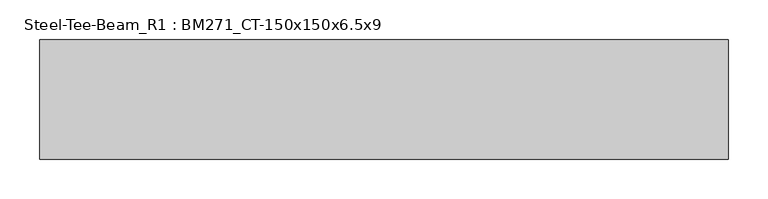
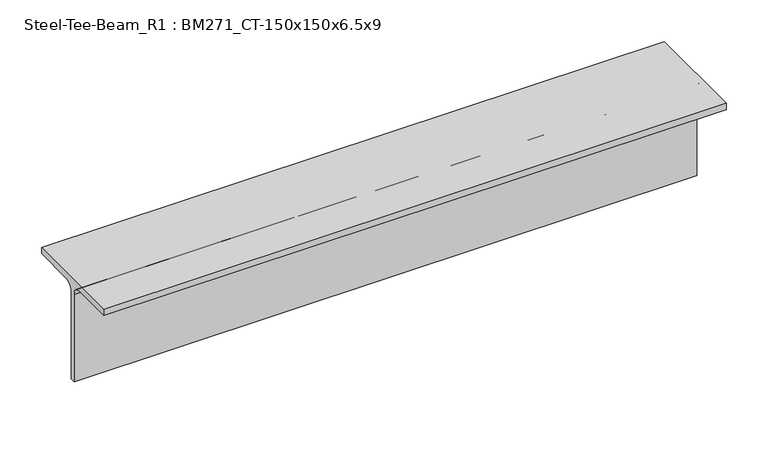
"""IFC4 building model written with IfcOpenShell, lengths in millimetres: member geometry, Steel-Tee-Beam_R1 : BM271_CT-150x150x6.5x9."""

from ifc_helpers import new_model, si_unit, point, frame, frame_2d, origin, place, context, project, spatial, polyline, circle_curve, trimmed, segment, composite_curve, outline, extrude, source, transform, mapped, element, save


def steel_tee_beam_r1_bm271_ct_150x150x6_5x9_bb86e743(model_context):
    return source(origin(), model_context, "Body", "SweptSolid", [
        extrude(outline(composite_curve([segment(polyline([(-75.0, 75.0), (75.0, 75.0), (75.0, 66.0), (16.25, 66.0)]), True, "CONTINUOUS"), segment(trimmed(circle_curve(frame_2d((16.25, 53.0)), 13.0), [point((16.25, 66.0))], [point((3.25, 53.0))], True, "CARTESIAN"), True, "CONTINUOUS"), segment(polyline([(3.25, 53.0), (3.25, -75.0), (-3.25, -75.0), (-3.25, 53.0)]), True, "CONTINUOUS"), segment(trimmed(circle_curve(frame_2d((-16.25, 53.0)), 13.0), [point((-3.25, 53.0))], [point((-16.25, 66.0))], True, "CARTESIAN"), True, "CONTINUOUS"), segment(polyline([(-16.25, 66.0), (-75.0, 66.0), (-75.0, 75.0)]), True, "CONTINUOUS")], self_intersect=False)), frame((-500.0, 0.0, 0.0), z_axis=(1.0, 0.0, 0.0), x_axis=(0.0, 1.0, 0.0)), (0.0, 0.0, 1.0), 865.9474508),
    ])


if __name__ == "__main__":
    model = new_model("IFC4")
    model_context = context("Model", 3, world=origin())
    ifc_project = project(units=[si_unit("LENGTHUNIT", "METRE", prefix="MILLI")], contexts=[model_context])
    site = spatial("IfcSite", under=ifc_project)
    building = spatial("IfcBuilding", under=site)
    placement = place(None, origin())
    steel_tee_beam_r1_bm271_ct_150x150x6_5x9_shape = steel_tee_beam_r1_bm271_ct_150x150x6_5x9_bb86e743(model_context)
    element("IfcMember", 1, ObjectType="Steel-Tee-Beam_R1 : BM271_CT-150x150x6.5x9", at=placement, inside=building, context=model_context, shape_type="MappedRepresentation", body=[
        mapped(steel_tee_beam_r1_bm271_ct_150x150x6_5x9_shape, transform((0.0, 0.0, 0.0), x_axis=(1.0, 0.0, 0.0), y_axis=(0.0, 1.0, 0.0), z_axis=(0.0, 0.0, 1.0))),
    ])
    save(model, "model.ifc")

# Revit data of these elements
# Type "Steel-Tee-Beam_R1 : BM271_CT-150x150x6.5x9"
#   Keynote = "CT-150x150x6.5x9"
#   Surface Area = 0.588841 m²/m
#   Section Area = 23.3904 cm²
#   Mass per Unit Length = 18.3614 kg/m
#   Length [instance default] = 1.5240 m
#   bf = 0.1500 m
#   d = 0.1500 m
#   k = 0.0220 m
#   r = 0.0130 m
#   tf = 0.0090 m
#   tw = 0.0065 m
#   hec_material4 [instance default] = none
#   hec_material3 [instance default] = none
#   hec_material2 [instance default] = none
#   hec_material1 [instance default] = none
#   Structural Material [instance default] = Steel, 45-345
#   Assembly Code = ""
# Element 1 (IfcMember, "Steel-Tee-Beam_R1 : BM271_CT-150x150x6.5x9")
#   Structural Material = none
# Materials
#   "Steel, 45-345": class "Metal", colour RGB 189 187 185, transparency 0, Description = "Steel 345 MPa", Cost = 0
